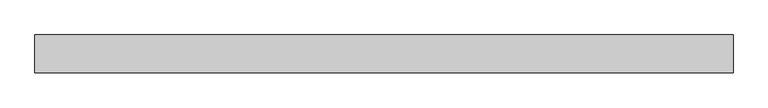
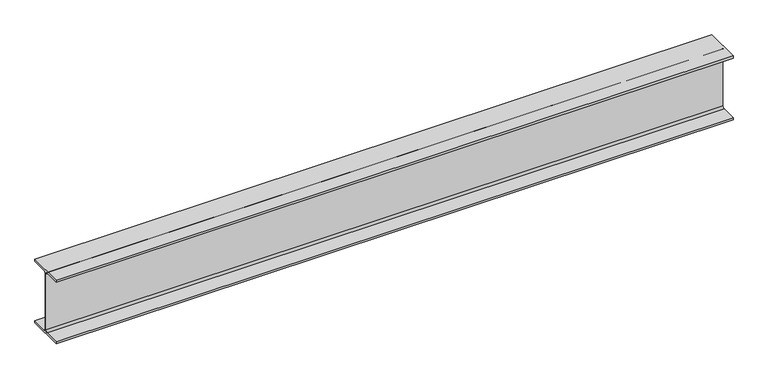
"""IFC4 building model written with IfcOpenShell, lengths in millimetres: beam geometry, Old_Steel Beam_H-KSD3502 : H_SB_ASB_H-200×200x8x12."""

from ifc_helpers import new_model, si_unit, point, frame, frame_2d, origin, place, context, project, spatial, polyline, circle_curve, trimmed, segment, composite_curve, outline, extrude, source, transform, mapped, element, save


def beam_363e02a8(model_context):
    return source(origin(), model_context, "Body", "SweptSolid", [
        extrude(outline(composite_curve([segment(polyline([(82.5, -141.5), (82.5, -151.7), (-82.5, -151.7), (-82.5, -141.5), (-11.9, -141.5)]), True, "CONTINUOUS"), segment(trimmed(circle_curve(frame_2d((-11.9, -132.6)), 8.9), [point((-11.9, -141.5))], [point((-3.0, -132.6))], True, "CARTESIAN"), True, "CONTINUOUS"), segment(polyline([(-3.0, -132.6), (-3.0, 132.6)]), True, "CONTINUOUS"), segment(trimmed(circle_curve(frame_2d((-11.9, 132.6)), 8.9), [point((-3.0, 132.6))], [point((-11.9, 141.5))], True, "CARTESIAN"), True, "CONTINUOUS"), segment(polyline([(-11.9, 141.5), (-82.5, 141.5), (-82.5, 151.7), (82.5, 151.7), (82.5, 141.5), (11.9, 141.5)]), True, "CONTINUOUS"), segment(trimmed(circle_curve(frame_2d((11.9, 132.6)), 8.9), [point((11.9, 141.5))], [point((3.0, 132.6))], True, "CARTESIAN"), True, "CONTINUOUS"), segment(polyline([(3.0, 132.6), (3.0, -132.6)]), True, "CONTINUOUS"), segment(trimmed(circle_curve(frame_2d((11.9, -132.6)), 8.9), [point((3.0, -132.6))], [point((11.9, -141.5))], True, "CARTESIAN"), True, "CONTINUOUS"), segment(polyline([(11.9, -141.5), (82.5, -141.5)]), True, "CONTINUOUS")], self_intersect=False)), frame((-1338.0077267, 0.0, 0.0), z_axis=(1.0, 0.0, 0.0), x_axis=(0.0, 1.0, 0.0)), (0.0, 0.0, 1.0), 3043.2161654),
    ])


if __name__ == "__main__":
    model = new_model("IFC4")
    model_context = context("Model", 3, world=origin())
    ifc_project = project(units=[si_unit("LENGTHUNIT", "METRE", prefix="MILLI")], contexts=[model_context])
    site = spatial("IfcSite", under=ifc_project)
    building = spatial("IfcBuilding", under=site)
    placement = place(None, origin())
    beam_shape = beam_363e02a8(model_context)
    element("IfcBeam", 1, ObjectType="Old_Steel Beam_H-KSD3502 : H_SB_ASB_H-200×200x8x12", at=placement, inside=building, context=model_context, shape_type="MappedRepresentation", body=[
        mapped(beam_shape, transform((0.0, 0.0, 0.0), x_axis=(1.0, 0.0, 0.0), y_axis=(0.0, 1.0, 0.0), z_axis=(0.0, 0.0, 1.0))),
    ])
    save(model, "model.ifc")

# Revit data of these elements
# Type "Old_Steel Beam_H-KSD3502 : H_SB_ASB_H-200×200x8x12"
#   Width = 20.0 cm
#   Web Thickness = 0.8 cm
#   Web Fillet = 1.3 cm
#   Warping Constant = 141376.0 cm⁶
#   Torsional Moment of Inertia = 26.2485 cm⁴
#   Torsional Modulus = 1.0 cm³
#   Section Area = 63.53 cm²
#   Plastic Modulus weak axis = 244.0 cm³
#   Plastic Modulus strong axis = 525.0 cm³
#   Perimeter = 1.16 m²/m
#   Nominal Weight = 49.90 kgf/m
#   Moment of Inertia weak axis = 1600.00 cm⁴
#   Moment of Inertia strong axis = 4720.00 cm⁴
#   Height = 20.0 cm
#   Flange Thickness = 1.2 cm
#   Elastic Modulus weak axis = 160.0 cm³
#   Elastic Modulus strong axis = 472.0 cm³
#   Centroid Vertical = 10.0 cm
#   Centroid Horizontal = 10.0 cm
#   Length [instance default] = 1.5240 m
#   Structural Material [instance default] = Steel, 45-345
#   Assembly Code = ""
# Element 1 (IfcBeam, "Old_Steel Beam_H-KSD3502 : H_SB_ASB_H-200×200x8x12")
#   Structural Material = none
# Materials
#   "Steel, 45-345": class "Metal", colour RGB 189 187 185, transparency 0, Description = "Steel 345 MPa", Cost = 0
